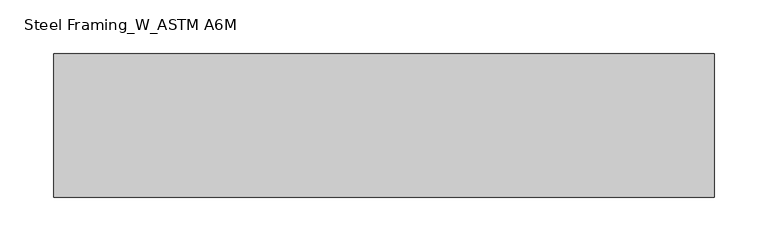
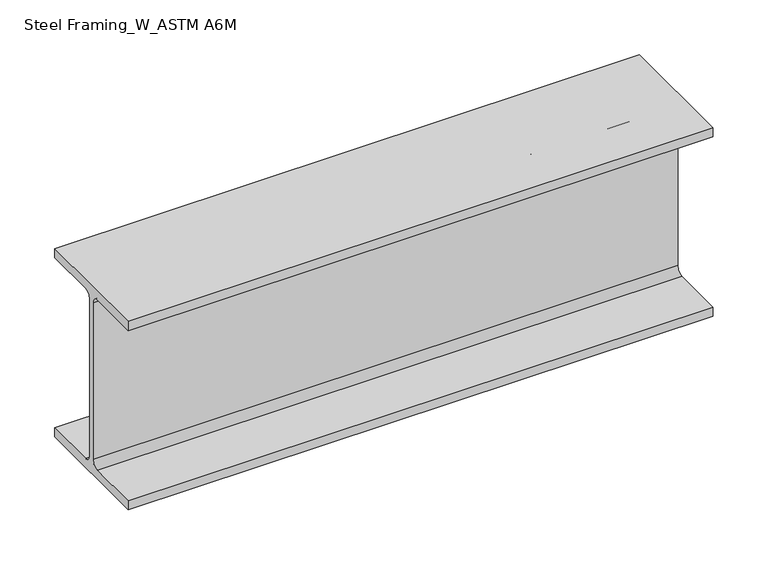
"""IFC4 building model written with IfcOpenShell, lengths in millimetres: beam geometry, Steel Framing_W_ASTM A6M : H_SB_AR_S02_W200x31.3_B6."""

import ifcopenshell
import ifcopenshell.guid

model = None  # the IFC model being written
_history = None  # IfcOwnerHistory: only IFC2X3 demands one
_inside = {}  # id of a spatial element -> (the spatial element, [elements in it])
_under = {}  # id of a project, library or spatial element -> (it, [spatial elements below it])
_declared = {}  # id of a project -> (the project, [libraries it declares])
_typed = {}  # id of a type object -> (the type object, [elements of that type])
_made_of = {}  # id of a material, layer set ... -> (it, [elements and type objects made of it])


def new_model(schema):
    """Start an empty IFC model of exactly this schema.

    Asked for "IFC4X3", IfcOpenShell would pick the latest addendum, in which some entities
    have other attributes; the version numbers below select the first issue.
    IFC2X3 requires an IfcOwnerHistory on every rooted entity: one is made here for all.
    """
    global model, _history
    if schema == "IFC4X3":
        model = ifcopenshell.file(schema_version=(4, 3, 0, 0))
    else:
        model = ifcopenshell.file(schema=schema)
    _inside.clear()
    _under.clear()
    _declared.clear()
    _typed.clear()
    _made_of.clear()
    _history = None
    if model.schema == "IFC2X3":
        org = make("IfcOrganization", Name="unknown")
        user = make(
            "IfcPersonAndOrganization",
            ThePerson=make("IfcPerson", FamilyName="unknown"),
            TheOrganization=org,
        )
        app = make(
            "IfcApplication",
            ApplicationDeveloper=org,
            Version="unknown",
            ApplicationFullName="unknown",
            ApplicationIdentifier="unknown",
        )
        _history = make(
            "IfcOwnerHistory",
            OwningUser=user,
            OwningApplication=app,
            ChangeAction="ADDED",
            CreationDate=0,
        )
    return model


def make(cls, **values):
    """One entity of the class cls with the attributes given. An attribute that is None is left unset."""
    return model.create_entity(
        cls, **{name: value for name, value in values.items() if value is not None}
    )


def rooted(cls, **values):
    """An entity with a GlobalId (a new one), such as an element, a storey or a relation."""
    return make(cls, GlobalId=ifcopenshell.guid.new(), OwnerHistory=_history, **values)


def si_unit(unit_type, name, prefix=None):
    """IfcSIUnit, for example si_unit("LENGTHUNIT", "METRE", prefix="MILLI")."""
    return make("IfcSIUnit", UnitType=unit_type, Prefix=prefix, Name=name)


def assignment(units):
    """IfcUnitAssignment: the units of a project."""
    return None if units is None else make("IfcUnitAssignment", Units=units)


def point(xyz):
    """IfcCartesianPoint."""
    return None if xyz is None else make("IfcCartesianPoint", Coordinates=xyz)


def direction(xyz):
    """IfcDirection."""
    return None if xyz is None else make("IfcDirection", DirectionRatios=xyz)


def frame(location, z_axis=None, x_axis=None):
    """IfcAxis2Placement3D, a coordinate frame: its origin and axes. An axis left out is left unset."""
    return make(
        "IfcAxis2Placement3D",
        Location=point(location),
        Axis=direction(z_axis),
        RefDirection=direction(x_axis),
    )


def frame_2d(location, x_axis=None):
    """IfcAxis2Placement2D, a coordinate frame in the plane: its origin and x axis."""
    return make(
        "IfcAxis2Placement2D", Location=point(location), RefDirection=direction(x_axis)
    )


def origin():
    """The frame at (0, 0, 0) with its axes left unset."""
    return frame((0.0, 0.0, 0.0))


def place(relative_to, where):
    """IfcLocalPlacement: puts the frame where relative to a parent placement (None: the world)."""
    return make(
        "IfcLocalPlacement", PlacementRelTo=relative_to, RelativePlacement=where
    )


def context(
    kind, dimensions, precision=None, world=None, true_north=None, identifier=None
):
    """IfcGeometricRepresentationContext, for example the 3D "Model" context."""
    return make(
        "IfcGeometricRepresentationContext",
        ContextIdentifier=identifier,
        ContextType=kind,
        CoordinateSpaceDimension=dimensions,
        Precision=precision,
        WorldCoordinateSystem=world,
        TrueNorth=true_north,
    )


def project(units=None, contexts=None):
    """IfcProject with its units and contexts."""
    return rooted(
        "IfcProject",
        Name="project",
        RepresentationContexts=contexts,
        UnitsInContext=assignment(units),
    )


def spatial(cls, under=None, at=None, **own):
    """A site, building, storey or space (cls), placed at a placement, below another one or the project."""
    s = rooted(cls, ObjectPlacement=at, **own)
    if under is not None:
        _under.setdefault(under.id(), (under, []))[1].append(s)
    return s


def polyline(points):
    """IfcPolyline through the points."""
    return make("IfcPolyline", Points=[point(p) for p in points])


def circle_curve(where, radius):
    """IfcCircle in the frame where."""
    return make("IfcCircle", Position=where, Radius=radius)


def trimmed(basis, trim1, trim2, sense, master):
    """IfcTrimmedCurve: the piece of a basis curve between two trims."""
    return make(
        "IfcTrimmedCurve",
        BasisCurve=basis,
        Trim1=trim1,
        Trim2=trim2,
        SenseAgreement=sense,
        MasterRepresentation=master,
    )


def segment(curve, same_sense, transition):
    """IfcCompositeCurveSegment."""
    return make(
        "IfcCompositeCurveSegment",
        Transition=transition,
        SameSense=same_sense,
        ParentCurve=curve,
    )


def composite_curve(segments, self_intersect=None):
    """IfcCompositeCurve: segments joined end to end."""
    return make("IfcCompositeCurve", Segments=segments, SelfIntersect=self_intersect)


def outline(outer, holes=None, kind="AREA"):
    """IfcArbitraryClosedProfileDef: a profile drawn as a closed curve; with holes, ...WithVoids."""
    if holes is None:
        return make("IfcArbitraryClosedProfileDef", ProfileType=kind, OuterCurve=outer)
    return make(
        "IfcArbitraryProfileDefWithVoids",
        ProfileType=kind,
        OuterCurve=outer,
        InnerCurves=holes,
    )


def extrude(swept, where, along, depth):
    """IfcExtrudedAreaSolid: the profile swept, set in the frame where, extruded along a direction by depth."""
    return make(
        "IfcExtrudedAreaSolid",
        SweptArea=swept,
        Position=where,
        ExtrudedDirection=direction(along),
        Depth=depth,
    )


def shape(context_of_items, identifier, shape_type, items):
    """IfcShapeRepresentation: the items that make up one representation, for example the "Body"."""
    return make(
        "IfcShapeRepresentation",
        ContextOfItems=context_of_items,
        RepresentationIdentifier=identifier,
        RepresentationType=shape_type,
        Items=items,
    )


def source(mapping_origin, context_of_items, identifier, shape_type, items):
    """IfcRepresentationMap: a shape defined once, which mapped items show again and again."""
    return make(
        "IfcRepresentationMap",
        MappingOrigin=mapping_origin,
        MappedRepresentation=shape(context_of_items, identifier, shape_type, items),
    )


def transform(
    local_origin,
    x_axis=None,
    y_axis=None,
    z_axis=None,
    scale=None,
    scale2=None,
    scale3=None,
    uniform=True,
):
    """IfcCartesianTransformationOperator3D, or its non-uniform kind. x_axis, y_axis, z_axis: its Axis1, 2, 3."""
    if uniform:
        return make(
            "IfcCartesianTransformationOperator3D",
            Axis1=direction(x_axis),
            Axis2=direction(y_axis),
            LocalOrigin=point(local_origin),
            Scale=scale,
            Axis3=direction(z_axis),
        )
    return make(
        "IfcCartesianTransformationOperator3DnonUniform",
        Axis1=direction(x_axis),
        Axis2=direction(y_axis),
        LocalOrigin=point(local_origin),
        Scale=scale,
        Axis3=direction(z_axis),
        Scale2=scale2,
        Scale3=scale3,
    )


def mapped(mapping_source, mapping_target):
    """IfcMappedItem: shows the shape of a source again, moved by a transform."""
    return make(
        "IfcMappedItem", MappingSource=mapping_source, MappingTarget=mapping_target
    )


def made_of(thing, what):
    """Note that an element or type object is made of a material, layer set ...; save() writes the relation."""
    if what is not None:
        _made_of.setdefault(what.id(), (what, []))[1].append(thing)
    return thing


def element(
    cls,
    number,
    at=None,
    inside=None,
    cuts=None,
    type_object=None,
    material=None,
    context=None,
    identifier="Body",
    shape_type=None,
    held_by="IfcProductDefinitionShape",
    body=None,
    shapes=None,
    **own,
):
    """One element of the class cls, such as IfcWall. Its Tag is "e" and its number.

    at: its placement. inside: the storey or other place that contains it. cuts: it is an
    opening in that element (IfcRelVoidsElement). A single representation is given by context,
    identifier, shape_type and body (its items); several are given by shapes. held_by: the class
    of the entity that holds the representations. save() writes the other relations.
    """
    e = rooted(cls, Tag="e%d" % number, ObjectPlacement=at, **own)
    if body is not None:
        shapes = [shape(context, identifier, shape_type, body)]
    if shapes is not None:
        e.Representation = make(held_by, Representations=shapes)
    if inside is not None:
        _inside.setdefault(inside.id(), (inside, []))[1].append(e)
    if cuts is not None:
        rooted(
            "IfcRelVoidsElement", RelatingBuildingElement=cuts, RelatedOpeningElement=e
        )
    if type_object is not None:
        _typed.setdefault(type_object.id(), (type_object, []))[1].append(e)
    return made_of(e, material)


def aggregate(whole, parts):
    """IfcRelAggregates: a whole, such as a stair, and the parts it consists of."""
    return rooted("IfcRelAggregates", RelatingObject=whole, RelatedObjects=parts)


def save(model, path):
    """Write the relations noted so far, then the file.

    IfcRelAggregates (storeys below a building ...), IfcRelContainedInSpatialStructure (elements
    in a storey), IfcRelDefinesByType, IfcRelAssociatesMaterial and IfcRelDeclares: one each for
    every whole, place, type object, material and project.
    """
    for whole, parts in _under.values():
        aggregate(whole, parts)
    for where, things in _inside.values():
        rooted(
            "IfcRelContainedInSpatialStructure",
            RelatedElements=things,
            RelatingStructure=where,
        )
    for kind, things in _typed.values():
        rooted("IfcRelDefinesByType", RelatedObjects=things, RelatingType=kind)
    for what, things in _made_of.values():
        rooted("IfcRelAssociatesMaterial", RelatedObjects=things, RelatingMaterial=what)
    for by, libraries in _declared.values():
        rooted("IfcRelDeclares", RelatingContext=by, RelatedDefinitions=libraries)
    model.write(path)


def steel_framing_w_astm_a6m_676d03db(model_context):
    return source(origin(), model_context, "Body", "SweptSolid", [
        extrude(outline(composite_curve([segment(polyline([(67.0, -94.8), (67.0, -105.0), (-67.0, -105.0), (-67.0, -94.8), (-10.775, -94.8)]), True, "CONTINUOUS"), segment(trimmed(circle_curve(frame_2d((-10.775, -87.2)), 7.6), [point((-10.775, -94.8))], [point((-3.175, -87.2))], True, "CARTESIAN"), True, "CONTINUOUS"), segment(polyline([(-3.175, -87.2), (-3.175, 87.2)]), True, "CONTINUOUS"), segment(trimmed(circle_curve(frame_2d((-10.775, 87.2)), 7.6), [point((-3.175, 87.2))], [point((-10.775, 94.8))], True, "CARTESIAN"), True, "CONTINUOUS"), segment(polyline([(-10.775, 94.8), (-67.0, 94.8), (-67.0, 105.0), (67.0, 105.0), (67.0, 94.8), (10.775, 94.8)]), True, "CONTINUOUS"), segment(trimmed(circle_curve(frame_2d((10.775, 87.2)), 7.6), [point((10.775, 94.8))], [point((3.175, 87.2))], True, "CARTESIAN"), True, "CONTINUOUS"), segment(polyline([(3.175, 87.2), (3.175, -87.2)]), True, "CONTINUOUS"), segment(trimmed(circle_curve(frame_2d((10.775, -87.2)), 7.6), [point((3.175, -87.2))], [point((10.775, -94.8))], True, "CARTESIAN"), True, "CONTINUOUS"), segment(polyline([(10.775, -94.8), (67.0, -94.8)]), True, "CONTINUOUS")], self_intersect=False)), frame((-345.3, 0.0, 0.0), z_axis=(1.0, 0.0, 0.0), x_axis=(0.0, 1.0, 0.0)), (0.0, 0.0, 1.0), 616.6),
    ])


if __name__ == "__main__":
    model = new_model("IFC4")
    model_context = context("Model", 3, world=origin())
    ifc_project = project(units=[si_unit("LENGTHUNIT", "METRE", prefix="MILLI")], contexts=[model_context])
    site = spatial("IfcSite", under=ifc_project)
    building = spatial("IfcBuilding", under=site)
    placement = place(None, origin())
    steel_framing_w_astm_a6m_shape = steel_framing_w_astm_a6m_676d03db(model_context)
    element("IfcBeam", 1, ObjectType="Steel Framing_W_ASTM A6M : H_SB_AR_S02_W200x31.3_B6", at=placement, inside=building, context=model_context, shape_type="MappedRepresentation", body=[
        mapped(steel_framing_w_astm_a6m_shape, transform((0.0, 0.0, 0.0), x_axis=(1.0, 0.0, 0.0), y_axis=(0.0, 1.0, 0.0), z_axis=(0.0, 0.0, 1.0))),
    ])
    save(model, "model.ifc")

# Revit data of these elements
# Type "Steel Framing_W_ASTM A6M : H_SB_AR_S02_W200x31.3_B6"
#   Type Mark = "B6"
#   Section Name Key = "W8x21"
#   Width = 13.4 cm
#   Web Thickness = 0.635 cm
#   Web Fillet = 0.76 cm
#   Warping Constant = 40800.0 cm⁶
#   Torsional Moment of Inertia = 11.70 cm⁴
#   Section Area = 39.7 cm²
#   Plastic Modulus weak axis = 93.2 cm³
#   Plastic Modulus strong axis = 334.0 cm³
#   Perimeter = 0.93 m²/m
#   Nominal Weight = 31.30 kgf/m
#   Moment of Inertia weak axis = 407.00 cm⁴
#   Moment of Inertia strong axis = 3130.00 cm⁴
#   Height = 21.0 cm
#   Flange Thickness = 1.02 cm
#   Elastic Modulus weak axis = 60.8 cm³
#   Elastic Modulus strong axis = 298.0 cm³
#   Centroid Vertical = 10.5 cm
#   Centroid Horizontal = 6.7 cm
#   Length [instance default] = 1500 mm
#   Structural Material [instance default] = Steel, 45-345
#   Bolt Spacing = 0
#   Assembly Code = ""
# Element 1 (IfcBeam, "Steel Framing_W_ASTM A6M : H_SB_AR_S02_W200x31.3_B6")
#   Materials on its faces: "Steel, 45-345"
# Materials
#   "Steel, 45-345": class "Metal", colour RGB 189 187 185, transparency 0, Description = "Steel 345 MPa", Cost = 0
